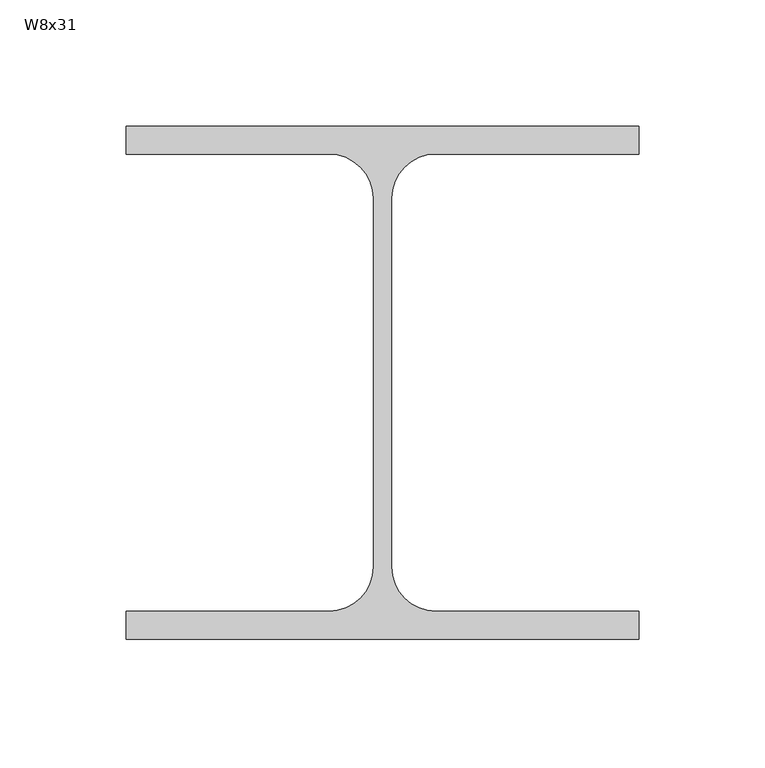
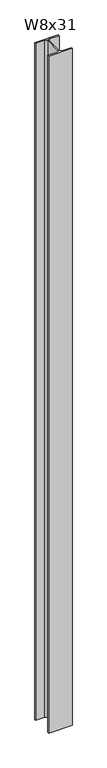
"""IFC4 building model written with IfcOpenShell, lengths in millimetres: column geometry, RME WF - Column : W8x31."""

from ifc_helpers import new_model, si_unit, point, frame, frame_2d, origin, place, context, project, spatial, polyline, circle_curve, trimmed, segment, composite_curve, outline, extrude, source, transform, mapped, element, save


def w8x31_c223d7c0(model_context):
    return source(origin(), model_context, "Body", "SweptSolid", [
        extrude(outline(composite_curve([segment(polyline([(101.6, 101.6), (101.6, 90.551), (21.1455, 90.551)]), True, "CONTINUOUS"), segment(trimmed(circle_curve(frame_2d((21.1455, 73.025)), 17.526), [point((21.1455, 90.551))], [point((3.6195, 73.025))], True, "CARTESIAN"), True, "CONTINUOUS"), segment(polyline([(3.6195, 73.025), (3.6195, -73.025)]), True, "CONTINUOUS"), segment(trimmed(circle_curve(frame_2d((21.1455, -73.025)), 17.526), [point((3.6195, -73.025))], [point((21.1455, -90.551))], True, "CARTESIAN"), True, "CONTINUOUS"), segment(polyline([(21.1455, -90.551), (101.6, -90.551), (101.6, -101.6), (-101.6, -101.6), (-101.6, -90.551), (-21.1455, -90.551)]), True, "CONTINUOUS"), segment(trimmed(circle_curve(frame_2d((-21.1455, -73.025)), 17.526), [point((-21.1455, -90.551))], [point((-3.6195, -73.025))], True, "CARTESIAN"), True, "CONTINUOUS"), segment(polyline([(-3.6195, -73.025), (-3.6195, 73.025)]), True, "CONTINUOUS"), segment(trimmed(circle_curve(frame_2d((-21.1455, 73.025)), 17.526), [point((-3.6195, 73.025))], [point((-21.1455, 90.551))], True, "CARTESIAN"), True, "CONTINUOUS"), segment(polyline([(-21.1455, 90.551), (-101.6, 90.551), (-101.6, 101.6), (101.6, 101.6)]), True, "CONTINUOUS")], self_intersect=False)), frame((0.0, 0.0, -304.8), z_axis=(0.0, 0.0, 1.0), x_axis=(1.0, 0.0, 0.0)), (0.0, 0.0, 1.0), 6172.2),
    ])


if __name__ == "__main__":
    model = new_model("IFC4")
    model_context = context("Model", 3, world=origin())
    ifc_project = project(units=[si_unit("LENGTHUNIT", "METRE", prefix="MILLI")], contexts=[model_context])
    site = spatial("IfcSite", under=ifc_project)
    building = spatial("IfcBuilding", under=site)
    placement = place(None, origin())
    w8x31_shape = w8x31_c223d7c0(model_context)
    element("IfcColumn", 1, ObjectType="RME WF - Column : W8x31", at=placement, inside=building, context=model_context, shape_type="MappedRepresentation", body=[
        mapped(w8x31_shape, transform((0.0, 0.0, 0.0), x_axis=(1.0, 0.0, 0.0), y_axis=(0.0, 1.0, 0.0), z_axis=(0.0, 0.0, 1.0))),
    ])
    save(model, "model.ifc")

# Revit data of these elements
# Type "RME WF - Column : W8x31"
#   REINF TYPE [instance default] = ""
#   Nominal Size = "W16"
#   COL REMARKS [instance default] = ""
#   BP [instance default] = ""
#   Assembly Code = "B10"
#   W = 31
#   bf = 0' - 8"
#   d = 0' - 8"
#   k = 0' - 1 1/8"
#   kr = 0' - 0.69"
#   tf = 0' - 0.435"
#   tw = 0' - 0.285"
#   A = 0.0633333 SF
#   Structural Material [instance default] = Metal - Steel - ASTM A992
# Element 1 (IfcColumn, "RME WF - Column : W8x31")
#   Materials on its faces: "Metal - Steel - ASTM A992"
# Materials
#   "Metal - Steel - ASTM A992": class "Metal", colour RGB 255 128 0, transparency 0
